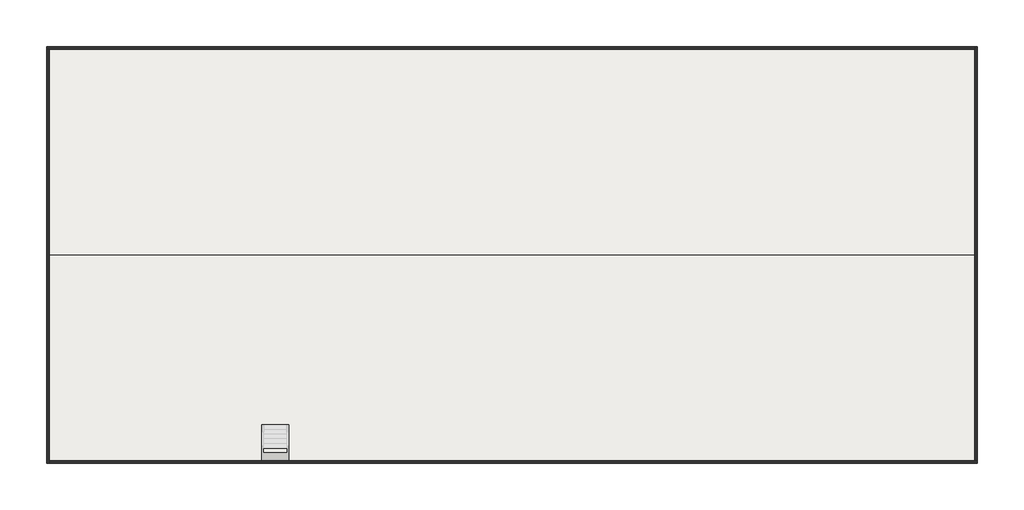
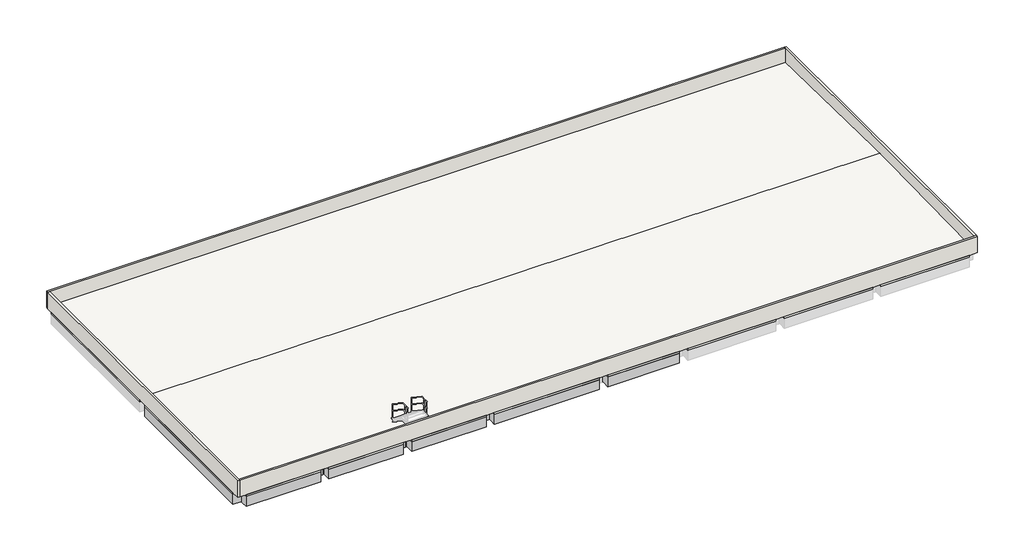
# One storey, part 1 of 3: 16 beams, 4 walls, 1 roof, 1 slab.
"""IFC4 building model written with IfcOpenShell, lengths in millimetres."""

from ifc_helpers import new_model, si_unit, frame, origin, place, context, project, spatial, polyline, outline, extrude, faceted_brep, element, save

model = new_model("IFC4")

# Units and contexts
model_context = context("Model", 3, world=origin())
ifc_project = project(units=[si_unit("LENGTHUNIT", "METRE", prefix="MILLI")], contexts=[model_context])

# Site, building, storey
site = spatial("IfcSite", under=ifc_project)
building = spatial("IfcBuilding", under=site)
storey = spatial("IfcBuildingStorey", under=building, Name="TOC", Elevation=7649.9618634)

# Beams
placement = place(None, origin())
element("IfcBeam", 1, ObjectType="RC Beam_Rectangular : H_SB_AR_S16_B600xH900_RG4", at=placement, inside=storey, context=model_context, shape_type="Brep", body=[
    faceted_brep([(300.0, 12499.5208589, 6749.9618634), (300.0, 12099.5208589, 6749.9618634), (300.0, 11899.5208589, 6749.9618634), (300.0, 11899.5208589, 7499.9618634), (300.0, 12499.5208589, 7499.9618634), (5700.0, 11899.5208589, 6749.9618634), (5700.0, 12099.5208589, 6749.9618634), (5700.0, 12499.5208589, 6749.9618634), (5700.0, 12499.5208589, 7499.9618634), (5700.0, 11899.5208589, 7499.9618634), (426.0, 11899.5208589, 7499.9618634), (2800.0, 11899.5208589, 7499.9618634), (3200.0, 11899.5208589, 7499.9618634), (3200.0, 12499.5208589, 7499.9618634), (2800.0, 12499.5208589, 7499.9618634), (426.0, 12499.5208589, 7499.9618634), (2800.0, 11899.5208589, 6749.9618634), (3200.0, 11899.5208589, 6749.9618634), (426.0, 12499.5208589, 6749.9618634), (2800.0, 12499.5208589, 6749.9618634), (3200.0, 12499.5208589, 6749.9618634)], [[[0, 1, 2, 3, 4]], [[5, 6, 7, 8, 9]], [[4, 3, 10, 11, 12, 9, 8, 13, 14, 15]], [[2, 16, 17, 5, 9, 12, 11, 10, 3]], [[2, 1, 0, 18, 19, 20, 7, 6, 5, 17, 16]], [[7, 20, 19, 18, 0, 4, 15, 14, 13, 8]]]),
])
element("IfcBeam", 2, ObjectType="RC Beam_Rectangular : H_SB_AR_S16_B600xH900_RG4", at=placement, inside=storey, context=model_context, shape_type="Brep", body=[
    faceted_brep([(6300.0, 12499.5208589, 6749.9618634), (6300.0, 12099.5208589, 6749.9618634), (6300.0, 11899.5208589, 6749.9618634), (6300.0, 11899.5208589, 7499.9618634), (6300.0, 12499.5208589, 7499.9618634), (11700.0, 11899.5208589, 6749.9618634), (11700.0, 12099.5208589, 6749.9618634), (11700.0, 12499.5208589, 6749.9618634), (11700.0, 12499.5208589, 7499.9618634), (11700.0, 11899.5208589, 7499.9618634), (8800.0, 11899.5208589, 7499.9618634), (9200.0, 11899.5208589, 7499.9618634), (9200.0, 12499.5208589, 7499.9618634), (8800.0, 12499.5208589, 7499.9618634), (8800.0, 11899.5208589, 6749.9618634), (9200.0, 11899.5208589, 6749.9618634), (8800.0, 12499.5208589, 6749.9618634), (9200.0, 12499.5208589, 6749.9618634)], [[[0, 1, 2, 3, 4]], [[5, 6, 7, 8, 9]], [[4, 3, 10, 11, 9, 8, 12, 13]], [[2, 14, 15, 5, 9, 11, 10, 3]], [[2, 1, 0, 16, 17, 7, 6, 5, 15, 14]], [[7, 17, 16, 0, 4, 13, 12, 8]]]),
])
element("IfcBeam", 3, ObjectType="RC Beam_Rectangular : H_SB_AR_S16_B600xH900_RG4", at=placement, inside=storey, context=model_context, shape_type="Brep", body=[
    faceted_brep([(12300.0, 12499.5208589, 6749.9618634), (12300.0, 12099.5208589, 6749.9618634), (12300.0, 11899.5208589, 6749.9618634), (12300.0, 11899.5208589, 7499.9618634), (12300.0, 12499.5208589, 7499.9618634), (17700.0, 11899.5208589, 6749.9618634), (17700.0, 12099.5208589, 6749.9618634), (17700.0, 12499.5208589, 6749.9618634), (17700.0, 12499.5208589, 7499.9618634), (17700.0, 11899.5208589, 7499.9618634), (14800.0, 11899.5208589, 7499.9618634), (15200.0, 11899.5208589, 7499.9618634), (15200.0, 12499.5208589, 7499.9618634), (14800.0, 12499.5208589, 7499.9618634), (14800.0, 11899.5208589, 6749.9618634), (15200.0, 11899.5208589, 6749.9618634), (14800.0, 12499.5208589, 6749.9618634), (15200.0, 12499.5208589, 6749.9618634)], [[[0, 1, 2, 3, 4]], [[5, 6, 7, 8, 9]], [[4, 3, 10, 11, 9, 8, 12, 13]], [[2, 14, 15, 5, 9, 11, 10, 3]], [[2, 1, 0, 16, 17, 7, 6, 5, 15, 14]], [[7, 17, 16, 0, 4, 13, 12, 8]]]),
])
element("IfcBeam", 4, ObjectType="RC Beam_Rectangular : H_SB_AR_S16_B600xH900_RG9", at=placement, inside=storey, context=model_context, shape_type="Brep", body=[
    faceted_brep([(300.0, 799.5208589, 6749.9618634), (300.0, 649.5208589, 6749.9618634), (300.0, 199.5208589, 6749.9618634), (300.0, 199.5208589, 7499.9618634), (300.0, 799.5208589, 7499.9618634), (5700.0, 199.5208589, 6749.9618634), (5700.0, 649.5208589, 6749.9618634), (5700.0, 799.5208589, 6749.9618634), (5700.0, 799.5208589, 7499.9618634), (5700.0, 199.5208589, 7499.9618634), (3200.0, 799.5208589, 7499.9618634), (2800.0, 799.5208589, 7499.9618634), (426.0, 799.5208589, 7499.9618634), (2800.0, 799.5208589, 6749.9618634), (3200.0, 799.5208589, 6749.9618634)], [[[0, 1, 2, 3, 4]], [[5, 6, 7, 8, 9]], [[4, 3, 9, 8, 10, 11, 12]], [[2, 5, 9, 3]], [[2, 1, 0, 13, 14, 7, 6, 5]], [[7, 14, 13, 0, 4, 12, 11, 10, 8]]]),
])
element("IfcBeam", 5, ObjectType="RC Beam_Rectangular : H_SB_AR_S16_B600xH900_RG9", at=placement, inside=storey, context=model_context, shape_type="Brep", body=[
    faceted_brep([(6300.0, 799.5208589, 6749.9618634), (6300.0, 649.5208589, 6749.9618634), (6300.0, 199.5208589, 6749.9618634), (6300.0, 199.5208589, 7499.9618634), (6300.0, 799.5208589, 7499.9618634), (11700.0, 199.5208589, 6749.9618634), (11700.0, 649.5208589, 6749.9618634), (11700.0, 799.5208589, 6749.9618634), (11700.0, 799.5208589, 7499.9618634), (11700.0, 199.5208589, 7499.9618634), (9200.0, 799.5208589, 7499.9618634), (8800.0, 799.5208589, 7499.9618634), (8800.0, 799.5208589, 6749.9618634), (9200.0, 799.5208589, 6749.9618634)], [[[0, 1, 2, 3, 4]], [[5, 6, 7, 8, 9]], [[4, 3, 9, 8, 10, 11]], [[2, 5, 9, 3]], [[2, 1, 0, 12, 13, 7, 6, 5]], [[7, 13, 12, 0, 4, 11, 10, 8]]]),
])
element("IfcBeam", 6, ObjectType="RC Beam_Rectangular : H_SB_AR_S16_B600xH900_RG9", at=placement, inside=storey, context=model_context, shape_type="Brep", body=[
    faceted_brep([(12300.0, 799.5208589, 6749.9618634), (12300.0, 649.5208589, 6749.9618634), (12300.0, 199.5208589, 6749.9618634), (12300.0, 199.5208589, 7499.9618634), (12300.0, 799.5208589, 7499.9618634), (17700.0, 199.5208589, 6749.9618634), (17700.0, 649.5208589, 6749.9618634), (17700.0, 799.5208589, 6749.9618634), (17700.0, 799.5208589, 7499.9618634), (17700.0, 199.5208589, 7499.9618634), (15200.0, 799.5208589, 7499.9618634), (14800.0, 799.5208589, 7499.9618634), (14800.0, 799.5208589, 6749.9618634), (15200.0, 799.5208589, 6749.9618634)], [[[0, 1, 2, 3, 4]], [[5, 6, 7, 8, 9]], [[4, 3, 9, 8, 10, 11]], [[2, 5, 9, 3]], [[2, 1, 0, 12, 13, 7, 6, 5]], [[7, 13, 12, 0, 4, 11, 10, 8]]]),
])
element("IfcBeam", 7, ObjectType="RC Beam_Rectangular : H_SB_AR_S16_B600xH900_RG9", at=placement, inside=storey, context=model_context, shape_type="Brep", body=[
    faceted_brep([(18300.0, 799.5208589, 6749.9618634), (18300.0, 649.5208589, 6749.9618634), (18300.0, 199.5208589, 6749.9618634), (18300.0, 199.5208589, 7499.9618634), (18300.0, 799.5208589, 7499.9618634), (25900.0, 199.5208589, 6749.9618634), (25900.0, 649.5208589, 6749.9618634), (25900.0, 799.5208589, 6749.9618634), (25900.0, 799.5208589, 7499.9618634), (25900.0, 199.5208589, 7499.9618634), (22400.0, 799.5208589, 7499.9618634), (21800.0, 799.5208589, 7499.9618634), (21800.0, 799.5208589, 6749.9618634), (22400.0, 799.5208589, 6749.9618634)], [[[0, 1, 2, 3, 4]], [[5, 6, 7, 8, 9]], [[4, 3, 9, 8, 10, 11]], [[2, 5, 9, 3]], [[2, 1, 0, 12, 13, 7, 6, 5]], [[7, 13, 12, 0, 4, 11, 10, 8]]]),
])
element("IfcBeam", 8, ObjectType="RC Beam_Rectangular : H_SB_AR_S16_B600xH900_RG9", at=placement, inside=storey, context=model_context, shape_type="Brep", body=[
    faceted_brep([(26500.0, 799.5208589, 6749.9618634), (26500.0, 649.5208589, 6749.9618634), (26500.0, 199.5208589, 6749.9618634), (26500.0, 199.5208589, 7499.9618634), (26500.0, 799.5208589, 7499.9618634), (31700.0, 199.5208589, 6749.9618634), (31700.0, 649.5208589, 6749.9618634), (31700.0, 799.5208589, 6749.9618634), (31700.0, 799.5208589, 7499.9618634), (31700.0, 199.5208589, 7499.9618634), (29400.0, 799.5208589, 7499.9618634), (28800.0, 799.5208589, 7499.9618634), (28700.0, 799.5208589, 7499.9618634), (28500.0, 799.5208589, 7499.9618634), (27855.0, 799.5208589, 7499.9618634), (26724.0, 799.5208589, 7499.9618634), (28800.0, 799.5208589, 6749.9618634), (29400.0, 799.5208589, 6749.9618634)], [[[0, 1, 2, 3, 4]], [[5, 6, 7, 8, 9]], [[4, 3, 9, 8, 10, 11, 12, 13, 14, 15]], [[2, 5, 9, 3]], [[2, 1, 0, 16, 17, 7, 6, 5]], [[7, 17, 16, 0, 4, 15, 14, 13, 12, 11, 10, 8]]]),
])
element("IfcBeam", 9, ObjectType="RC Beam_Rectangular : H_SB_AR_S16_B600xH900_RG6", at=placement, inside=storey, context=model_context, shape_type="Brep", body=[
    faceted_brep([(300.0, 11899.5208589, 6749.9618634), (150.0, 11899.5208589, 6749.9618634), (-300.0, 11899.5208589, 6749.9618634), (-300.0, 11899.5208589, 7499.9618634), (300.0, 11899.5208589, 7499.9618634), (-300.0, 799.5208589, 6749.9618634), (150.0, 799.5208589, 6749.9618634), (300.0, 799.5208589, 6749.9618634), (300.0, 799.5208589, 7499.9618634), (-300.0, 799.5208589, 7499.9618634)], [[[0, 1, 2, 3, 4]], [[5, 6, 7, 8, 9]], [[4, 3, 9, 8]], [[7, 0, 4, 8]], [[2, 1, 0, 7, 6, 5]], [[2, 5, 9, 3]]]),
])
element("IfcBeam", 10, ObjectType="RC Beam_Rectangular : H_SB_AR_S16_B400xH900_RG1", at=placement, inside=storey, context=model_context, shape_type="Brep", body=[
    faceted_brep([(5800.0, 799.5208589, 7499.9618634), (6200.0, 799.5208589, 7499.9618634), (6200.0, 925.5208589, 7499.9618634), (6200.0, 11899.5208589, 7499.9618634), (5800.0, 11899.5208589, 7499.9618634), (5800.0, 925.5208589, 7499.9618634), (5800.0, 799.5208589, 6749.9618634), (6200.0, 799.5208589, 6749.9618634), (6200.0, 11899.5208589, 6749.9618634), (5800.0, 11899.5208589, 6749.9618634), (6200.0, 925.5208589, 6749.9618634), (5800.0, 925.5208589, 6749.9618634)], [[[0, 1, 2, 3, 4, 5]], [[6, 7, 1, 0]], [[8, 9, 4, 3]], [[7, 10, 8, 3, 2, 1]], [[6, 11, 9, 8, 10, 7]], [[9, 11, 6, 0, 5, 4]]]),
])
element("IfcBeam", 11, ObjectType="RC Beam_Rectangular : H_SB_AR_S16_B400xH900_RG1", at=placement, inside=storey, context=model_context, shape_type="Brep", body=[
    faceted_brep([(11800.0, 799.5208589, 7499.9618634), (12200.0, 799.5208589, 7499.9618634), (12200.0, 925.5208589, 7499.9618634), (12200.0, 11899.5208589, 7499.9618634), (11800.0, 11899.5208589, 7499.9618634), (11800.0, 925.5208589, 7499.9618634), (11800.0, 799.5208589, 6749.9618634), (12200.0, 799.5208589, 6749.9618634), (12200.0, 11899.5208589, 6749.9618634), (11800.0, 11899.5208589, 6749.9618634), (12200.0, 925.5208589, 6749.9618634), (11800.0, 925.5208589, 6749.9618634)], [[[0, 1, 2, 3, 4, 5]], [[6, 7, 1, 0]], [[8, 9, 4, 3]], [[7, 10, 8, 3, 2, 1]], [[6, 11, 9, 8, 10, 7]], [[9, 11, 6, 0, 5, 4]]]),
])
element("IfcBeam", 12, ObjectType="RC Beam_Rectangular : H_SB_AR_S16_B600xH900_RG1A", at=placement, inside=storey, context=model_context, shape_type="Brep", body=[
    faceted_brep([(17700.0, 799.5208589, 7499.9618634), (18300.0, 799.5208589, 7499.9618634), (18300.0, 925.5208589, 7499.9618634), (18300.0, 7999.5208589, 7499.9618634), (18300.0, 8599.5208589, 7499.9618634), (18300.0, 11899.5208589, 7499.9618634), (17700.0, 11899.5208589, 7499.9618634), (17700.0, 925.5208589, 7499.9618634), (17700.0, 799.5208589, 6749.9618634), (18100.0, 799.5208589, 6749.9618634), (18300.0, 799.5208589, 6749.9618634), (18300.0, 11899.5208589, 6749.9618634), (18100.0, 11899.5208589, 6749.9618634), (17700.0, 11899.5208589, 6749.9618634), (18300.0, 7999.5208589, 6749.9618634), (18300.0, 8599.5208589, 6749.9618634), (17700.0, 925.5208589, 6749.9618634)], [[[0, 1, 2, 3, 4, 5, 6, 7]], [[8, 9, 10, 1, 0]], [[11, 12, 13, 6, 5]], [[10, 14, 15, 11, 5, 4, 3, 2, 1]], [[8, 16, 13, 12, 11, 15, 14, 10, 9]], [[13, 16, 8, 0, 7, 6]]]),
])
element("IfcBeam", 13, ObjectType="RC Beam_Rectangular : H_SB_AR_S16_B400xH900_RB1", at=placement, inside=storey, context=model_context, shape_type="Brep", body=[
    faceted_brep([(2800.0, 11899.5208589, 6749.9618634), (2800.0, 925.5208589, 6749.9618634), (2800.0, 799.5208589, 6749.9618634), (2800.0, 799.5208589, 7499.9618634), (2800.0, 925.5208589, 7499.9618634), (2800.0, 11899.5208589, 7499.9618634), (3200.0, 11899.5208589, 6749.9618634), (3200.0, 925.5208589, 6749.9618634), (3200.0, 799.5208589, 6749.9618634), (3200.0, 11899.5208589, 7499.9618634), (3200.0, 925.5208589, 7499.9618634), (3200.0, 799.5208589, 7499.9618634)], [[[0, 1, 2, 3, 4, 5]], [[0, 6, 7, 8, 2, 1]], [[8, 7, 6, 9, 10, 11]], [[6, 0, 5, 9]], [[2, 8, 11, 3]], [[5, 4, 3, 11, 10, 9]]]),
])
element("IfcBeam", 14, ObjectType="RC Beam_Rectangular : H_SB_AR_S16_B400xH900_RB1", at=placement, inside=storey, context=model_context, shape_type="Brep", body=[
    faceted_brep([(8800.0, 11899.5208589, 6749.9618634), (8800.0, 925.5208589, 6749.9618634), (8800.0, 799.5208589, 6749.9618634), (8800.0, 799.5208589, 7499.9618634), (8800.0, 925.5208589, 7499.9618634), (8800.0, 11899.5208589, 7499.9618634), (9200.0, 11899.5208589, 6749.9618634), (9200.0, 925.5208589, 6749.9618634), (9200.0, 799.5208589, 6749.9618634), (9200.0, 11899.5208589, 7499.9618634), (9200.0, 925.5208589, 7499.9618634), (9200.0, 799.5208589, 7499.9618634)], [[[0, 1, 2, 3, 4, 5]], [[0, 6, 7, 8, 2, 1]], [[8, 7, 6, 9, 10, 11]], [[6, 0, 5, 9]], [[2, 8, 11, 3]], [[5, 4, 3, 11, 10, 9]]]),
])
element("IfcBeam", 15, ObjectType="RC Beam_Rectangular : H_SB_AR_S16_B400xH900_RB1", at=placement, inside=storey, context=model_context, shape_type="Brep", body=[
    faceted_brep([(14800.0, 11899.5208589, 6749.9618634), (14800.0, 925.5208589, 6749.9618634), (14800.0, 799.5208589, 6749.9618634), (14800.0, 799.5208589, 7499.9618634), (14800.0, 925.5208589, 7499.9618634), (14800.0, 11899.5208589, 7499.9618634), (15200.0, 11899.5208589, 6749.9618634), (15200.0, 925.5208589, 6749.9618634), (15200.0, 799.5208589, 6749.9618634), (15200.0, 11899.5208589, 7499.9618634), (15200.0, 925.5208589, 7499.9618634), (15200.0, 799.5208589, 7499.9618634)], [[[0, 1, 2, 3, 4, 5]], [[0, 6, 7, 8, 2, 1]], [[8, 7, 6, 9, 10, 11]], [[6, 0, 5, 9]], [[2, 8, 11, 3]], [[5, 4, 3, 11, 10, 9]]]),
])
element("IfcBeam", 16, ObjectType="RC Beam_Rectangular : H_SB_AR_S16_B600xH900_RB3", at=placement, inside=storey, context=model_context, shape_type="Brep", body=[
    faceted_brep([(21800.0, 7999.5208589, 6749.9618634), (21800.0, 925.5208589, 6749.9618634), (21800.0, 799.5208589, 6749.9618634), (21800.0, 799.5208589, 7499.9618634), (21800.0, 925.5208589, 7499.9618634), (21800.0, 7999.5208589, 7499.9618634), (22400.0, 7999.5208589, 6749.9618634), (22400.0, 925.5208589, 6749.9618634), (22400.0, 799.5208589, 6749.9618634), (22400.0, 7999.5208589, 7499.9618634), (22400.0, 925.5208589, 7499.9618634), (22400.0, 799.5208589, 7499.9618634)], [[[0, 1, 2, 3, 4, 5]], [[0, 6, 7, 8, 2, 1]], [[8, 7, 6, 9, 10, 11]], [[6, 0, 5, 9]], [[2, 8, 11, 3]], [[5, 4, 3, 11, 10, 9]]]),
])

# Roof
element("IfcRoof", 17, ObjectType="H_RF_AR_B06_Mortar(Slope)_XPS_Memb_T50+120", at=placement, inside=storey, context=model_context, shape_type="SweptSolid", body=[
    extrude(outline(polyline([(24049.5208589, 7821.4618634), (24049.5208589, 7649.9618634), (349.5208589, 7649.9618634), (349.5208589, 7821.4618634), (12199.5208589, 8054.4618634), (24049.5208589, 7821.4618634)])), frame((-150.0, 0.0, 0.0), z_axis=(1.0, 0.0, 0.0), x_axis=(0.0, 1.0, 0.0)), (0.0, 0.0, 1.0), 53300.0),
])

# Slab
element("IfcSlab", 18, ObjectType="H_FL_AR_S17_Roof RC Slab_T150", at=placement, inside=storey, context=model_context, shape_type="Brep", body=[
    faceted_brep([(300.0, 11899.5208589, 7499.9618634), (300.0, 12499.5208589, 7499.9618634), (-300.0, 12499.5208589, 7499.9618634), (-300.0, 23599.5208589, 7499.9618634), (300.0, 23599.5208589, 7499.9618634), (300.0, 24199.5208589, 7499.9618634), (5700.0, 24199.5208589, 7499.9618634), (5700.0, 23599.5208589, 7499.9618634), (5800.0, 23599.5208589, 7499.9618634), (6200.0, 23599.5208589, 7499.9618634), (6300.0, 23599.5208589, 7499.9618634), (6300.0, 24199.5208589, 7499.9618634), (11700.0, 24199.5208589, 7499.9618634), (11700.0, 23599.5208589, 7499.9618634), (11800.0, 23599.5208589, 7499.9618634), (12200.0, 23599.5208589, 7499.9618634), (12300.0, 23599.5208589, 7499.9618634), (12300.0, 24199.5208589, 7499.9618634), (17700.0, 24199.5208589, 7499.9618634), (17700.0, 23599.5208589, 7499.9618634), (18300.0, 23599.5208589, 7499.9618634), (18300.0, 24199.5208589, 7499.9618634), (25900.0, 24199.5208589, 7499.9618634), (25900.0, 23599.5208589, 7499.9618634), (25950.0, 23599.5208589, 7499.9618634), (26450.0, 23599.5208589, 7499.9618634), (26500.0, 23599.5208589, 7499.9618634), (26500.0, 24199.5208589, 7499.9618634), (31700.0, 24199.5208589, 7499.9618634), (31700.0, 23599.5208589, 7499.9618634), (31750.0, 23599.5208589, 7499.9618634), (32250.0, 23599.5208589, 7499.9618634), (32300.0, 23599.5208589, 7499.9618634), (32300.0, 24199.5208589, 7499.9618634), (38700.0, 24199.5208589, 7499.9618634), (38700.0, 23599.5208589, 7499.9618634), (38750.0, 23599.5208589, 7499.9618634), (39250.0, 23599.5208589, 7499.9618634), (39300.0, 23599.5208589, 7499.9618634), (39300.0, 24199.5208589, 7499.9618634), (45700.0, 24199.5208589, 7499.9618634), (45700.0, 23599.5208589, 7499.9618634), (45750.0, 23599.5208589, 7499.9618634), (46250.0, 23599.5208589, 7499.9618634), (46300.0, 23599.5208589, 7499.9618634), (46300.0, 24199.5208589, 7499.9618634), (52700.0, 24199.5208589, 7499.9618634), (52700.0, 23599.5208589, 7499.9618634), (53300.0, 23599.5208589, 7499.9618634), (53300.0, 8599.5208589, 7499.9618634), (52700.0, 8599.5208589, 7499.9618634), (52700.0, 7999.5208589, 7499.9618634), (53300.0, 7999.5208589, 7499.9618634), (53300.0, 799.5208589, 7499.9618634), (52700.0, 799.5208589, 7499.9618634), (52700.0, 199.5208589, 7499.9618634), (46300.0, 199.5208589, 7499.9618634), (46300.0, 799.5208589, 7499.9618634), (46250.0, 799.5208589, 7499.9618634), (45750.0, 799.5208589, 7499.9618634), (45700.0, 799.5208589, 7499.9618634), (45700.0, 199.5208589, 7499.9618634), (39300.0, 199.5208589, 7499.9618634), (39300.0, 799.5208589, 7499.9618634), (39250.0, 799.5208589, 7499.9618634), (38750.0, 799.5208589, 7499.9618634), (38700.0, 799.5208589, 7499.9618634), (38700.0, 199.5208589, 7499.9618634), (32300.0, 199.5208589, 7499.9618634), (32300.0, 799.5208589, 7499.9618634), (32250.0, 799.5208589, 7499.9618634), (31750.0, 799.5208589, 7499.9618634), (31700.0, 799.5208589, 7499.9618634), (31700.0, 199.5208589, 7499.9618634), (26500.0, 199.5208589, 7499.9618634), (26500.0, 799.5208589, 7499.9618634), (26450.0, 799.5208589, 7499.9618634), (25950.0, 799.5208589, 7499.9618634), (25900.0, 799.5208589, 7499.9618634), (25900.0, 199.5208589, 7499.9618634), (18300.0, 199.5208589, 7499.9618634), (18300.0, 799.5208589, 7499.9618634), (17700.0, 799.5208589, 7499.9618634), (17700.0, 199.5208589, 7499.9618634), (12300.0, 199.5208589, 7499.9618634), (12300.0, 799.5208589, 7499.9618634), (12200.0, 799.5208589, 7499.9618634), (11800.0, 799.5208589, 7499.9618634), (11700.0, 799.5208589, 7499.9618634), (11700.0, 199.5208589, 7499.9618634), (6300.0, 199.5208589, 7499.9618634), (6300.0, 799.5208589, 7499.9618634), (6200.0, 799.5208589, 7499.9618634), (5800.0, 799.5208589, 7499.9618634), (5700.0, 799.5208589, 7499.9618634), (5700.0, 199.5208589, 7499.9618634), (300.0, 199.5208589, 7499.9618634), (300.0, 799.5208589, 7499.9618634), (-300.0, 799.5208589, 7499.9618634), (-300.0, 11899.5208589, 7499.9618634), (18300.0, 11899.5208589, 7499.9618634), (18300.0, 12499.5208589, 7499.9618634), (17700.0, 12499.5208589, 7499.9618634), (17700.0, 11899.5208589, 7499.9618634), (6300.0, 11899.5208589, 7499.9618634), (6300.0, 12499.5208589, 7499.9618634), (6200.0, 12499.5208589, 7499.9618634), (5800.0, 12499.5208589, 7499.9618634), (5700.0, 12499.5208589, 7499.9618634), (5700.0, 11899.5208589, 7499.9618634), (5800.0, 11899.5208589, 7499.9618634), (6200.0, 11899.5208589, 7499.9618634), (12300.0, 11899.5208589, 7499.9618634), (12300.0, 12499.5208589, 7499.9618634), (12200.0, 12499.5208589, 7499.9618634), (11800.0, 12499.5208589, 7499.9618634), (11700.0, 12499.5208589, 7499.9618634), (11700.0, 11899.5208589, 7499.9618634), (11800.0, 11899.5208589, 7499.9618634), (12200.0, 11899.5208589, 7499.9618634), (26500.0, 7999.5208589, 7499.9618634), (26500.0, 8599.5208589, 7499.9618634), (26450.0, 8599.5208589, 7499.9618634), (25950.0, 8599.5208589, 7499.9618634), (25900.0, 8599.5208589, 7499.9618634), (25900.0, 7999.5208589, 7499.9618634), (25950.0, 7999.5208589, 7499.9618634), (26450.0, 7999.5208589, 7499.9618634), (32300.0, 7999.5208589, 7499.9618634), (32300.0, 8599.5208589, 7499.9618634), (32250.0, 8599.5208589, 7499.9618634), (31750.0, 8599.5208589, 7499.9618634), (31700.0, 8599.5208589, 7499.9618634), (31700.0, 7999.5208589, 7499.9618634), (31750.0, 7999.5208589, 7499.9618634), (32250.0, 7999.5208589, 7499.9618634), (39300.0, 7999.5208589, 7499.9618634), (39300.0, 8599.5208589, 7499.9618634), (39250.0, 8599.5208589, 7499.9618634), (38750.0, 8599.5208589, 7499.9618634), (38700.0, 8599.5208589, 7499.9618634), (38700.0, 7999.5208589, 7499.9618634), (38750.0, 7999.5208589, 7499.9618634), (39250.0, 7999.5208589, 7499.9618634), (46300.0, 7999.5208589, 7499.9618634), (46300.0, 8599.5208589, 7499.9618634), (46250.0, 8599.5208589, 7499.9618634), (45750.0, 8599.5208589, 7499.9618634), (45700.0, 8599.5208589, 7499.9618634), (45700.0, 7999.5208589, 7499.9618634), (45750.0, 7999.5208589, 7499.9618634), (46250.0, 7999.5208589, 7499.9618634), (300.0, 12499.5208589, 7649.9618634), (300.0, 11899.5208589, 7649.9618634), (-300.0, 11899.5208589, 7649.9618634), (-300.0, 799.5208589, 7649.9618634), (300.0, 799.5208589, 7649.9618634), (300.0, 199.5208589, 7649.9618634), (5700.0, 199.5208589, 7649.9618634), (5700.0, 799.5208589, 7649.9618634), (6300.0, 799.5208589, 7649.9618634), (6300.0, 199.5208589, 7649.9618634), (11700.0, 199.5208589, 7649.9618634), (11700.0, 799.5208589, 7649.9618634), (12300.0, 799.5208589, 7649.9618634), (12300.0, 199.5208589, 7649.9618634), (17700.0, 199.5208589, 7649.9618634), (17700.0, 799.5208589, 7649.9618634), (18300.0, 799.5208589, 7649.9618634), (18300.0, 199.5208589, 7649.9618634), (25900.0, 199.5208589, 7649.9618634), (25900.0, 799.5208589, 7649.9618634), (26500.0, 799.5208589, 7649.9618634), (26500.0, 199.5208589, 7649.9618634), (31700.0, 199.5208589, 7649.9618634), (31700.0, 799.5208589, 7649.9618634), (32300.0, 799.5208589, 7649.9618634), (32300.0, 199.5208589, 7649.9618634), (38700.0, 199.5208589, 7649.9618634), (38700.0, 799.5208589, 7649.9618634), (39300.0, 799.5208589, 7649.9618634), (39300.0, 199.5208589, 7649.9618634), (45700.0, 199.5208589, 7649.9618634), (45700.0, 799.5208589, 7649.9618634), (46300.0, 799.5208589, 7649.9618634), (46300.0, 199.5208589, 7649.9618634), (52700.0, 199.5208589, 7649.9618634), (52700.0, 799.5208589, 7649.9618634), (53300.0, 799.5208589, 7649.9618634), (53300.0, 7999.5208589, 7649.9618634), (52700.0, 7999.5208589, 7649.9618634), (52700.0, 8599.5208589, 7649.9618634), (53300.0, 8599.5208589, 7649.9618634), (53300.0, 23599.5208589, 7649.9618634), (52700.0, 23599.5208589, 7649.9618634), (52700.0, 24199.5208589, 7649.9618634), (46300.0, 24199.5208589, 7649.9618634), (46300.0, 23599.5208589, 7649.9618634), (45700.0, 23599.5208589, 7649.9618634), (45700.0, 24199.5208589, 7649.9618634), (39300.0, 24199.5208589, 7649.9618634), (39300.0, 23599.5208589, 7649.9618634), (38700.0, 23599.5208589, 7649.9618634), (38700.0, 24199.5208589, 7649.9618634), (32300.0, 24199.5208589, 7649.9618634), (32300.0, 23599.5208589, 7649.9618634), (31700.0, 23599.5208589, 7649.9618634), (31700.0, 24199.5208589, 7649.9618634), (26500.0, 24199.5208589, 7649.9618634), (26500.0, 23599.5208589, 7649.9618634), (25900.0, 23599.5208589, 7649.9618634), (25900.0, 24199.5208589, 7649.9618634), (18300.0, 24199.5208589, 7649.9618634), (18300.0, 23599.5208589, 7649.9618634), (17700.0, 23599.5208589, 7649.9618634), (17700.0, 24199.5208589, 7649.9618634), (12300.0, 24199.5208589, 7649.9618634), (12300.0, 23599.5208589, 7649.9618634), (11700.0, 23599.5208589, 7649.9618634), (11700.0, 24199.5208589, 7649.9618634), (6300.0, 24199.5208589, 7649.9618634), (6300.0, 23599.5208589, 7649.9618634), (5700.0, 23599.5208589, 7649.9618634), (5700.0, 24199.5208589, 7649.9618634), (300.0, 24199.5208589, 7649.9618634), (300.0, 23599.5208589, 7649.9618634), (-300.0, 23599.5208589, 7649.9618634), (-300.0, 12499.5208589, 7649.9618634), (6300.0, 12499.5208589, 7649.9618634), (6300.0, 11899.5208589, 7649.9618634), (5700.0, 11899.5208589, 7649.9618634), (5700.0, 12499.5208589, 7649.9618634), (12300.0, 12499.5208589, 7649.9618634), (12300.0, 11899.5208589, 7649.9618634), (11700.0, 11899.5208589, 7649.9618634), (11700.0, 12499.5208589, 7649.9618634), (18300.0, 12499.5208589, 7649.9618634), (18300.0, 11899.5208589, 7649.9618634), (17700.0, 11899.5208589, 7649.9618634), (17700.0, 12499.5208589, 7649.9618634), (26500.0, 8599.5208589, 7649.9618634), (26500.0, 7999.5208589, 7649.9618634), (25900.0, 7999.5208589, 7649.9618634), (25900.0, 8599.5208589, 7649.9618634), (32300.0, 8599.5208589, 7649.9618634), (32300.0, 7999.5208589, 7649.9618634), (31700.0, 7999.5208589, 7649.9618634), (31700.0, 8599.5208589, 7649.9618634), (39300.0, 8599.5208589, 7649.9618634), (39300.0, 7999.5208589, 7649.9618634), (38700.0, 7999.5208589, 7649.9618634), (38700.0, 8599.5208589, 7649.9618634), (46300.0, 8599.5208589, 7649.9618634), (46300.0, 7999.5208589, 7649.9618634), (45700.0, 7999.5208589, 7649.9618634), (45700.0, 8599.5208589, 7649.9618634)], [[[0, 1, 2, 3, 4, 5, 6, 7, 8, 9, 10, 11, 12, 13, 14, 15, 16, 17, 18, 19, 20, 21, 22, 23, 24, 25, 26, 27, 28, 29, 30, 31, 32, 33, 34, 35, 36, 37, 38, 39, 40, 41, 42, 43, 44, 45, 46, 47, 48, 49, 50, 51, 52, 53, 54, 55, 56, 57, 58, 59, 60, 61, 62, 63, 64, 65, 66, 67, 68, 69, 70, 71, 72, 73, 74, 75, 76, 77, 78, 79, 80, 81, 82, 83, 84, 85, 86, 87, 88, 89, 90, 91, 92, 93, 94, 95, 96, 97, 98, 99], [100, 101, 102, 103], [104, 105, 106, 107, 108, 109, 110, 111], [112, 113, 114, 115, 116, 117, 118, 119], [120, 121, 122, 123, 124, 125, 126, 127], [128, 129, 130, 131, 132, 133, 134, 135], [136, 137, 138, 139, 140, 141, 142, 143], [144, 145, 146, 147, 148, 149, 150, 151]], [[152, 153, 154, 155, 156, 157, 158, 159, 160, 161, 162, 163, 164, 165, 166, 167, 168, 169, 170, 171, 172, 173, 174, 175, 176, 177, 178, 179, 180, 181, 182, 183, 184, 185, 186, 187, 188, 189, 190, 191, 192, 193, 194, 195, 196, 197, 198, 199, 200, 201, 202, 203, 204, 205, 206, 207, 208, 209, 210, 211, 212, 213, 214, 215, 216, 217, 218, 219, 220, 221, 222, 223, 224, 225, 226, 227], [228, 229, 230, 231], [232, 233, 234, 235], [236, 237, 238, 239], [240, 241, 242, 243], [244, 245, 246, 247], [248, 249, 250, 251], [252, 253, 254, 255]], [[48, 193, 192, 49]], [[52, 189, 188, 53]], [[157, 96, 95, 158]], [[161, 90, 89, 162]], [[165, 84, 83, 166]], [[169, 80, 79, 170]], [[173, 74, 73, 174]], [[177, 68, 67, 178]], [[181, 62, 61, 182]], [[185, 56, 55, 186]], [[154, 99, 98, 155]], [[2, 227, 226, 3]], [[5, 224, 223, 6]], [[11, 220, 219, 12]], [[17, 216, 215, 18]], [[21, 212, 211, 22]], [[27, 208, 207, 28]], [[33, 204, 203, 34]], [[39, 200, 199, 40]], [[45, 196, 195, 46]], [[0, 153, 152, 1]], [[153, 0, 99, 154]], [[1, 152, 227, 2]], [[104, 229, 228, 105]], [[229, 104, 111, 110, 109, 230]], [[230, 109, 108, 231]], [[231, 108, 107, 106, 105, 228]], [[112, 233, 232, 113]], [[233, 112, 119, 118, 117, 234]], [[234, 117, 116, 235]], [[235, 116, 115, 114, 113, 232]], [[100, 237, 236, 101]], [[237, 100, 103, 238]], [[238, 103, 102, 239]], [[239, 102, 101, 236]], [[4, 225, 224, 5]], [[225, 4, 3, 226]], [[10, 221, 220, 11]], [[221, 10, 9, 8, 7, 222]], [[222, 7, 6, 223]], [[16, 217, 216, 17]], [[217, 16, 15, 14, 13, 218]], [[218, 13, 12, 219]], [[20, 213, 212, 21]], [[213, 20, 19, 214]], [[214, 19, 18, 215]], [[26, 209, 208, 27]], [[209, 26, 25, 24, 23, 210]], [[210, 23, 22, 211]], [[32, 205, 204, 33]], [[205, 32, 31, 30, 29, 206]], [[206, 29, 28, 207]], [[38, 201, 200, 39]], [[201, 38, 37, 36, 35, 202]], [[202, 35, 34, 203]], [[44, 197, 196, 45]], [[197, 44, 43, 42, 41, 198]], [[198, 41, 40, 199]], [[47, 194, 193, 48]], [[194, 47, 46, 195]], [[120, 241, 240, 121]], [[241, 120, 127, 126, 125, 242]], [[242, 125, 124, 243]], [[243, 124, 123, 122, 121, 240]], [[128, 245, 244, 129]], [[245, 128, 135, 134, 133, 246]], [[246, 133, 132, 247]], [[247, 132, 131, 130, 129, 244]], [[136, 249, 248, 137]], [[249, 136, 143, 142, 141, 250]], [[250, 141, 140, 251]], [[251, 140, 139, 138, 137, 248]], [[144, 253, 252, 145]], [[253, 144, 151, 150, 149, 254]], [[254, 149, 148, 255]], [[255, 148, 147, 146, 145, 252]], [[51, 190, 189, 52]], [[190, 51, 50, 191]], [[191, 50, 49, 192]], [[156, 97, 96, 157]], [[97, 156, 155, 98]], [[160, 91, 90, 161]], [[94, 159, 158, 95]], [[159, 94, 93, 92, 91, 160]], [[164, 85, 84, 165]], [[88, 163, 162, 89]], [[163, 88, 87, 86, 85, 164]], [[168, 81, 80, 169]], [[82, 167, 166, 83]], [[167, 82, 81, 168]], [[172, 75, 74, 173]], [[78, 171, 170, 79]], [[171, 78, 77, 76, 75, 172]], [[176, 69, 68, 177]], [[72, 175, 174, 73]], [[175, 72, 71, 70, 69, 176]], [[180, 63, 62, 181]], [[66, 179, 178, 67]], [[179, 66, 65, 64, 63, 180]], [[184, 57, 56, 185]], [[60, 183, 182, 61]], [[183, 60, 59, 58, 57, 184]], [[54, 187, 186, 55]], [[187, 54, 53, 188]]]),
])

# Walls
element("IfcWall", 19, ObjectType="H_WA_AR_B02_Ext Wall_RC T150", at=placement, inside=storey, context=model_context, shape_type="Brep", body=[
    faceted_brep([(-300.0, 24049.5208589, 7649.9618634), (-150.0, 24049.5208589, 7649.9618634), (53150.0, 24049.5208589, 7649.9618634), (53150.0, 24049.5208589, 7821.4618634), (53150.0, 24049.5208589, 8899.9618634), (-150.0, 24049.5208589, 8899.9618634), (-300.0, 24049.5208589, 8899.9618634), (-300.0, 24199.5208589, 7649.9618634), (-300.0, 24199.5208589, 8899.9618634), (53150.0, 24199.5208589, 8899.9618634), (53150.0, 24199.5208589, 7649.9618634), (52700.0, 24199.5208589, 7649.9618634), (46300.0, 24199.5208589, 7649.9618634), (45700.0, 24199.5208589, 7649.9618634), (39300.0, 24199.5208589, 7649.9618634), (38700.0, 24199.5208589, 7649.9618634), (32300.0, 24199.5208589, 7649.9618634), (31700.0, 24199.5208589, 7649.9618634), (26500.0, 24199.5208589, 7649.9618634), (25900.0, 24199.5208589, 7649.9618634), (18300.0, 24199.5208589, 7649.9618634), (17700.0, 24199.5208589, 7649.9618634), (12300.0, 24199.5208589, 7649.9618634), (11700.0, 24199.5208589, 7649.9618634), (6300.0, 24199.5208589, 7649.9618634), (5700.0, 24199.5208589, 7649.9618634), (300.0, 24199.5208589, 7649.9618634)], [[[0, 1, 2, 3, 4, 5, 6]], [[7, 8, 9, 10, 11, 12, 13, 14, 15, 16, 17, 18, 19, 20, 21, 22, 23, 24, 25, 26]], [[2, 1, 0, 7, 26, 25, 24, 23, 22, 21, 20, 19, 18, 17, 16, 15, 14, 13, 12, 11, 10]], [[6, 5, 4, 9, 8]], [[0, 6, 8, 7]], [[4, 3, 2, 10, 9]]]),
])
element("IfcWall", 20, ObjectType="H_WA_AR_B02_Ext Wall_RC T150", at=placement, inside=storey, context=model_context, shape_type="Brep", body=[
    faceted_brep([(-150.0, 199.5208589, 7649.9618634), (-150.0, 349.5208589, 7649.9618634), (-150.0, 24049.5208589, 7649.9618634), (-150.0, 24049.5208589, 7821.4618634), (-150.0, 24049.5208589, 8899.9618634), (-150.0, 349.5208589, 8899.9618634), (-150.0, 199.5208589, 8899.9618634), (-300.0, 199.5208589, 7649.9618634), (-300.0, 199.5208589, 8899.9618634), (-300.0, 24049.5208589, 8899.9618634), (-300.0, 24049.5208589, 7649.9618634), (-300.0, 23599.5208589, 7649.9618634), (-300.0, 12499.5208589, 7649.9618634), (-300.0, 11899.5208589, 7649.9618634), (-300.0, 799.5208589, 7649.9618634)], [[[0, 1, 2, 3, 4, 5, 6]], [[7, 8, 9, 10, 11, 12, 13, 14]], [[2, 1, 0, 7, 14, 13, 12, 11, 10]], [[6, 5, 4, 9, 8]], [[0, 6, 8, 7]], [[4, 3, 2, 10, 9]]]),
])
element("IfcWall", 21, ObjectType="H_WA_AR_B02_Ext Wall_RC T150", at=placement, inside=storey, context=model_context, shape_type="Brep", body=[
    faceted_brep([(53300.0, 349.5208589, 7649.9618634), (53150.0, 349.5208589, 7649.9618634), (-150.0, 349.5208589, 7649.9618634), (-150.0, 349.5208589, 7821.4618634), (-150.0, 349.5208589, 8899.9618634), (53150.0, 349.5208589, 8899.9618634), (53300.0, 349.5208589, 8899.9618634), (53300.0, 199.5208589, 7649.9618634), (53300.0, 199.5208589, 8899.9618634), (-150.0, 199.5208589, 8899.9618634), (-150.0, 199.5208589, 7649.9618634), (300.0, 199.5208589, 7649.9618634), (5700.0, 199.5208589, 7649.9618634), (6300.0, 199.5208589, 7649.9618634), (11700.0, 199.5208589, 7649.9618634), (12300.0, 199.5208589, 7649.9618634), (17700.0, 199.5208589, 7649.9618634), (18300.0, 199.5208589, 7649.9618634), (25900.0, 199.5208589, 7649.9618634), (26500.0, 199.5208589, 7649.9618634), (31700.0, 199.5208589, 7649.9618634), (32300.0, 199.5208589, 7649.9618634), (38700.0, 199.5208589, 7649.9618634), (39300.0, 199.5208589, 7649.9618634), (45700.0, 199.5208589, 7649.9618634), (46300.0, 199.5208589, 7649.9618634), (52700.0, 199.5208589, 7649.9618634)], [[[0, 1, 2, 3, 4, 5, 6]], [[7, 8, 9, 10, 11, 12, 13, 14, 15, 16, 17, 18, 19, 20, 21, 22, 23, 24, 25, 26]], [[2, 1, 0, 7, 26, 25, 24, 23, 22, 21, 20, 19, 18, 17, 16, 15, 14, 13, 12, 11, 10]], [[6, 5, 4, 9, 8]], [[0, 6, 8, 7]], [[4, 3, 2, 10, 9]]]),
])
element("IfcWall", 22, ObjectType="H_WA_AR_B02_Ext Wall_RC T150", at=placement, inside=storey, context=model_context, shape_type="Brep", body=[
    faceted_brep([(53150.0, 24199.5208589, 7649.9618634), (53150.0, 24049.5208589, 7649.9618634), (53150.0, 349.5208589, 7649.9618634), (53150.0, 349.5208589, 7821.4618634), (53150.0, 349.5208589, 8899.9618634), (53150.0, 24049.5208589, 8899.9618634), (53150.0, 24199.5208589, 8899.9618634), (53300.0, 24199.5208589, 7649.9618634), (53300.0, 24199.5208589, 8899.9618634), (53300.0, 349.5208589, 8899.9618634), (53300.0, 349.5208589, 7649.9618634), (53300.0, 799.5208589, 7649.9618634), (53300.0, 7999.5208589, 7649.9618634), (53300.0, 8599.5208589, 7649.9618634), (53300.0, 23599.5208589, 7649.9618634)], [[[0, 1, 2, 3, 4, 5, 6]], [[7, 8, 9, 10, 11, 12, 13, 14]], [[2, 1, 0, 7, 14, 13, 12, 11, 10]], [[6, 5, 4, 9, 8]], [[0, 6, 8, 7]], [[4, 3, 2, 10, 9]]]),
])

save(model, "model.ifc")

# Revit data of these elements
# Type "RC Beam_Rectangular : H_SB_AR_S16_B600xH900_RG4"
#   중앙부 하부근 = ""
#   중앙부 상부근 = ""
#   중앙부 보조근 = ""
#   중앙부 늑근 = ""
#   외단부 하부근 = ""
#   외단부 상부근 = ""
#   외단부 보조근 = ""
#   외단부 늑근 = ""
#   부호 = "TG3"
#   내단부 하부근 = ""
#   내단부 상부근 = ""
#   내단부 보조근 = ""
#   내단부 늑근 = ""
#   ALL 하부근 = "3-D20"
#   ALL 상부근 = "3-D20"
#   ALL 보조근 = ""
#   ALL 늑근 = "2-D10 @120"
#   Width = 600 mm
#   Height = 900 mm
#   Length [instance default] = 1524 mm
#   b = 600 mm
#   h = 900 mm
#   hec_material3 [instance default] = none
#   hec_material2 [instance default] = none
#   hec_material1 [instance default] = none
#   Structural Material [instance default] = none
#   Assembly Code = ""
# Type "RC Beam_Rectangular : H_SB_AR_S16_B600xH900_RG9"
#   중앙부 하부근 = ""
#   중앙부 상부근 = ""
#   중앙부 보조근 = ""
#   중앙부 늑근 = ""
#   외단부 하부근 = ""
#   외단부 상부근 = ""
#   외단부 보조근 = ""
#   외단부 늑근 = ""
#   부호 = "TG3"
#   내단부 하부근 = ""
#   내단부 상부근 = ""
#   내단부 보조근 = ""
#   내단부 늑근 = ""
#   ALL 하부근 = "3-D20"
#   ALL 상부근 = "3-D20"
#   ALL 보조근 = ""
#   ALL 늑근 = "2-D10 @120"
#   Width = 600 mm
#   Height = 900 mm
#   Length [instance default] = 1524 mm
#   b = 600 mm
#   h = 900 mm
#   hec_material3 [instance default] = none
#   hec_material2 [instance default] = none
#   hec_material1 [instance default] = none
#   Structural Material [instance default] = none
#   Assembly Code = ""
# Type "RC Beam_Rectangular : H_SB_AR_S16_B600xH900_RG6"
#   중앙부 하부근 = ""
#   중앙부 상부근 = ""
#   중앙부 보조근 = ""
#   중앙부 늑근 = ""
#   외단부 하부근 = ""
#   외단부 상부근 = ""
#   외단부 보조근 = ""
#   외단부 늑근 = ""
#   부호 = "TG3"
#   내단부 하부근 = ""
#   내단부 상부근 = ""
#   내단부 보조근 = ""
#   내단부 늑근 = ""
#   ALL 하부근 = "3-D20"
#   ALL 상부근 = "3-D20"
#   ALL 보조근 = ""
#   ALL 늑근 = "2-D10 @120"
#   Width = 600 mm
#   Height = 900 mm
#   Length [instance default] = 1524 mm
#   b = 600 mm
#   h = 900 mm
#   hec_material3 [instance default] = none
#   hec_material2 [instance default] = none
#   hec_material1 [instance default] = none
#   Structural Material [instance default] = none
#   Assembly Code = ""
# Type "RC Beam_Rectangular : H_SB_AR_S16_B400xH900_RG1"
#   중앙부 하부근 = ""
#   중앙부 상부근 = ""
#   중앙부 보조근 = ""
#   중앙부 늑근 = ""
#   외단부 하부근 = ""
#   외단부 상부근 = ""
#   외단부 보조근 = ""
#   외단부 늑근 = ""
#   부호 = "TG3"
#   내단부 하부근 = ""
#   내단부 상부근 = ""
#   내단부 보조근 = ""
#   내단부 늑근 = ""
#   ALL 하부근 = "3-D20"
#   ALL 상부근 = "3-D20"
#   ALL 보조근 = ""
#   ALL 늑근 = "2-D10 @120"
#   Width = 400 mm
#   Height = 900 mm
#   Length [instance default] = 1524 mm
#   b = 400 mm
#   h = 900 mm
#   hec_material3 [instance default] = none
#   hec_material2 [instance default] = none
#   hec_material1 [instance default] = none
#   Structural Material [instance default] = none
#   Assembly Code = ""
# Type "RC Beam_Rectangular : H_SB_AR_S16_B600xH900_RG1A"
#   중앙부 하부근 = ""
#   중앙부 상부근 = ""
#   중앙부 보조근 = ""
#   중앙부 늑근 = ""
#   외단부 하부근 = ""
#   외단부 상부근 = ""
#   외단부 보조근 = ""
#   외단부 늑근 = ""
#   부호 = "TG3"
#   내단부 하부근 = ""
#   내단부 상부근 = ""
#   내단부 보조근 = ""
#   내단부 늑근 = ""
#   ALL 하부근 = "3-D20"
#   ALL 상부근 = "3-D20"
#   ALL 보조근 = ""
#   ALL 늑근 = "2-D10 @120"
#   Width = 600 mm
#   Height = 900 mm
#   Length [instance default] = 1524 mm
#   b = 600 mm
#   h = 900 mm
#   hec_material3 [instance default] = none
#   hec_material2 [instance default] = none
#   hec_material1 [instance default] = none
#   Structural Material [instance default] = none
#   Assembly Code = ""
# Type "RC Beam_Rectangular : H_SB_AR_S16_B400xH900_RB1"
#   중앙부 하부근 = ""
#   중앙부 상부근 = ""
#   중앙부 보조근 = ""
#   중앙부 늑근 = ""
#   외단부 하부근 = ""
#   외단부 상부근 = ""
#   외단부 보조근 = ""
#   외단부 늑근 = ""
#   부호 = "TG3"
#   내단부 하부근 = ""
#   내단부 상부근 = ""
#   내단부 보조근 = ""
#   내단부 늑근 = ""
#   ALL 하부근 = "3-D20"
#   ALL 상부근 = "3-D20"
#   ALL 보조근 = ""
#   ALL 늑근 = "2-D10 @120"
#   Width = 400 mm
#   Height = 900 mm
#   Length [instance default] = 1524 mm
#   b = 400 mm
#   h = 900 mm
#   hec_material3 [instance default] = none
#   hec_material2 [instance default] = none
#   hec_material1 [instance default] = none
#   Structural Material [instance default] = none
#   Assembly Code = ""
# Type "RC Beam_Rectangular : H_SB_AR_S16_B600xH900_RB3"
#   중앙부 하부근 = ""
#   중앙부 상부근 = ""
#   중앙부 보조근 = ""
#   중앙부 늑근 = ""
#   외단부 하부근 = ""
#   외단부 상부근 = ""
#   외단부 보조근 = ""
#   외단부 늑근 = ""
#   부호 = "TG3"
#   내단부 하부근 = ""
#   내단부 상부근 = ""
#   내단부 보조근 = ""
#   내단부 늑근 = ""
#   ALL 하부근 = "3-D20"
#   ALL 상부근 = "3-D20"
#   ALL 보조근 = ""
#   ALL 늑근 = "2-D10 @120"
#   Width = 600 mm
#   Height = 900 mm
#   Length [instance default] = 1524 mm
#   b = 600 mm
#   h = 900 mm
#   hec_material3 [instance default] = none
#   hec_material2 [instance default] = none
#   hec_material1 [instance default] = none
#   Structural Material [instance default] = none
#   Assembly Code = ""
# Type "H_RF_AR_B06_Mortar(Slope)_XPS_Memb_T50+120"
#   Layers, outside or top first: 1.5 mm "Roofing - EPDM Membrane" (function 4); 120 mm "00_Insulation_Rigid_hec" (function 3); 50 mm "Slab, Screed" (function 1)
# Type "H_FL_AR_S17_Roof RC Slab_T150"
#   Keynote = ""
#   Type Comments = ""
#   Description = ""
#   Function = 1
#   Layers, outside or top first: 150 mm "Concrete - Cast-in-Place Concrete - 35 MPa" (function 1)
# Type "H_WA_AR_B02_Ext Wall_RC T150"
#   Type Comments = ""
#   Layers, outside or top first: 150 mm "Concrete - Cast-in-Place Concrete - 35 MPa" (function 1)
# Elements 1, 2, 3 (IfcBeam, "RC Beam_Rectangular : H_SB_AR_S16_B600xH900_RG4")
#   Comments = ""
#   hec_material3 = none
#   hec_material2 = none
#   hec_material1 = none
#   Structural Material = Concrete - Cast-in-Place Concrete - 35 MPa
#   Phase Created = New Construction
#   Materials on its faces: "Concrete - Cast-in-Place Concrete - 35 MPa"
# Elements 4, 5, 6, 7, 8 (IfcBeam, "RC Beam_Rectangular : H_SB_AR_S16_B600xH900_RG9")
#   Comments = ""
#   hec_material3 = none
#   hec_material2 = none
#   hec_material1 = none
#   Structural Material = Concrete - Cast-in-Place Concrete - 35 MPa
#   Phase Created = New Construction
#   Materials on its faces: "Concrete - Cast-in-Place Concrete - 35 MPa"
# Element 9 (IfcBeam, "RC Beam_Rectangular : H_SB_AR_S16_B600xH900_RG6")
#   Comments = ""
#   hec_material3 = none
#   hec_material2 = none
#   hec_material1 = none
#   Structural Material = Concrete - Cast-in-Place Concrete - 35 MPa
#   Phase Created = New Construction
#   Materials on its faces: "Concrete - Cast-in-Place Concrete - 35 MPa"
# Elements 10, 11 (IfcBeam, "RC Beam_Rectangular : H_SB_AR_S16_B400xH900_RG1")
#   Comments = ""
#   hec_material3 = none
#   hec_material2 = none
#   hec_material1 = none
#   Structural Material = Concrete - Cast-in-Place Concrete - 35 MPa
#   Phase Created = New Construction
#   Materials on its faces: "Concrete - Cast-in-Place Concrete - 35 MPa"
# Element 12 (IfcBeam, "RC Beam_Rectangular : H_SB_AR_S16_B600xH900_RG1A")
#   Comments = ""
#   hec_material3 = none
#   hec_material2 = none
#   hec_material1 = none
#   Structural Material = Concrete - Cast-in-Place Concrete - 35 MPa
#   Phase Created = New Construction
#   Materials on its faces: "Concrete - Cast-in-Place Concrete - 35 MPa"
# Elements 13, 14, 15 (IfcBeam, "RC Beam_Rectangular : H_SB_AR_S16_B400xH900_RB1")
#   hec_material3 = none
#   hec_material2 = none
#   hec_material1 = none
#   Structural Material = Concrete - Cast-in-Place Concrete - 35 MPa
#   Phase Created = New Construction
#   Materials on its faces: "Concrete - Cast-in-Place Concrete - 35 MPa"
# Element 16 (IfcBeam, "RC Beam_Rectangular : H_SB_AR_S16_B600xH900_RB3")
#   hec_material3 = none
#   hec_material2 = none
#   hec_material1 = none
#   Structural Material = Concrete - Cast-in-Place Concrete - 35 MPa
#   Phase Created = New Construction
#   Materials on its faces: "Concrete - Cast-in-Place Concrete - 35 MPa"
# Element 17 (IfcRoof, "H_RF_AR_B06_Mortar(Slope)_XPS_Memb_T50+120")
#   H_Roof Style Name = "Concrete Slab(Slope)+Insulation+Protection Concrete+Waterproofing"
#   H_Roof_Base Material = "Concrete Slab"
#   H_Roof_Finish-1 = "Liquid Waterproofing"
#   H_Roof_Finish-2 = "Rigid Extruded Polystyrene Foam Insulation(XPS)"
#   H_Roof_Finish-3 = "Welded Wire Fabric"
#   H_Roof_Finish-4 = "Protective Concrete w/ Steel Trowel Finish"
#   H_Roof_Finish-5 = "스카이패널 건식복합방수"
#   H_Roof_Style Remark = "* 스카이패널 건식복합방수 : WM 없음"
#   built-in parameter 1001705 = 25.661 (stored number, unit not read)
#   built-in parameter 1001710 = 33615
#   H_Roof Style No = RF41
#   Phase Created = New Construction
#   Materials on its faces: "Slab, Screed", "Roofing - EPDM Membrane"
# Element 18 (IfcSlab, "H_FL_AR_S17_Roof RC Slab_T150")
#   Comments = ""
#   TMP_Element Name = "SS2"
#   Height Offset From Level = 0 mm
#   built-in parameter 1001954 = 1
#   Phase Created = New Construction
#   Materials on its faces: "Concrete - Cast-in-Place Concrete - 35 MPa"
# Elements 19, 20, 21, 22 (IfcWall, "H_WA_AR_B02_Ext Wall_RC T150")
#   Top Offset = 0 mm
#   Base Offset = 0 mm
#   wall height = 1250 mm
#   Phase Created = New Construction
#   Base Constraint = TOC
#   Top Constraint = TOP
#   Materials on its faces: "Concrete - Cast-in-Place Concrete - 35 MPa"
# Materials
#   "Roofing - EPDM Membrane": class "Plastic", colour RGB 127 127 127, transparency 0, Description = "Exterior finish, roofing"
#   "00_Insulation_Rigid_hec": class "Insulation", colour RGB 255 255 217, transparency 0, Description = "Insulation(Rigid)", Cost = 0
#   "Slab, Screed": class "Concrete", colour RGB 120 120 120, transparency 0, Description = "Concrete slab topping", Cost = 0
#   "Concrete - Cast-in-Place Concrete - 35 MPa": class "Concrete", colour RGB 192 192 192, transparency 0, Cost = 0
